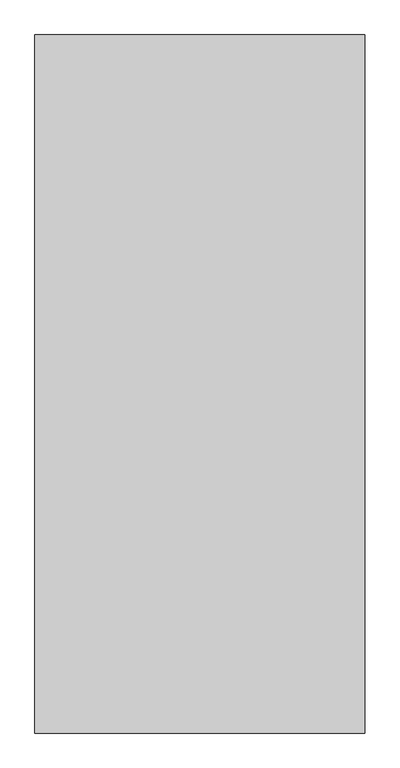
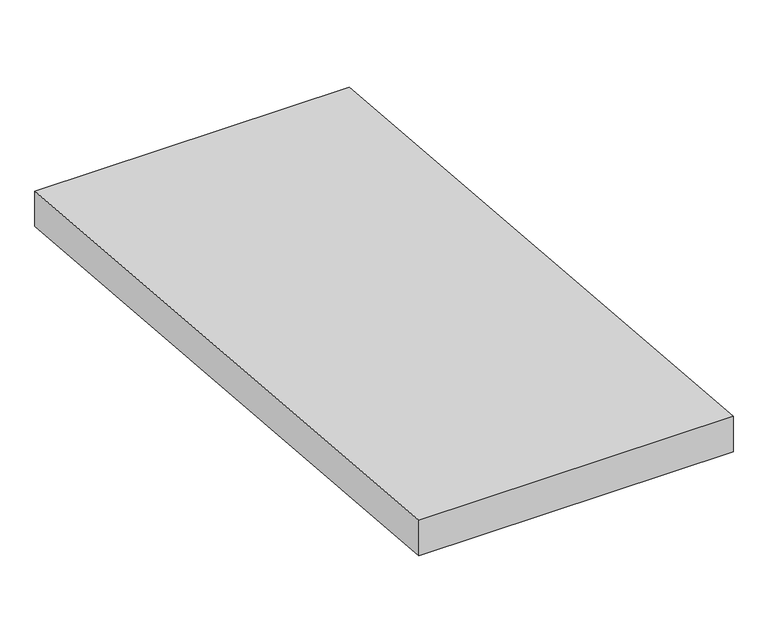
"""IFC4 building model written with IfcOpenShell, lengths in millimetres: ramp geometry."""

import ifcopenshell
import ifcopenshell.guid

model = None  # the IFC model being written
_history = None  # IfcOwnerHistory: only IFC2X3 demands one
_inside = {}  # id of a spatial element -> (the spatial element, [elements in it])
_under = {}  # id of a project, library or spatial element -> (it, [spatial elements below it])
_declared = {}  # id of a project -> (the project, [libraries it declares])
_typed = {}  # id of a type object -> (the type object, [elements of that type])
_made_of = {}  # id of a material, layer set ... -> (it, [elements and type objects made of it])


def new_model(schema):
    """Start an empty IFC model of exactly this schema.

    Asked for "IFC4X3", IfcOpenShell would pick the latest addendum, in which some entities
    have other attributes; the version numbers below select the first issue.
    IFC2X3 requires an IfcOwnerHistory on every rooted entity: one is made here for all.
    """
    global model, _history
    if schema == "IFC4X3":
        model = ifcopenshell.file(schema_version=(4, 3, 0, 0))
    else:
        model = ifcopenshell.file(schema=schema)
    _inside.clear()
    _under.clear()
    _declared.clear()
    _typed.clear()
    _made_of.clear()
    _history = None
    if model.schema == "IFC2X3":
        org = make("IfcOrganization", Name="unknown")
        user = make(
            "IfcPersonAndOrganization",
            ThePerson=make("IfcPerson", FamilyName="unknown"),
            TheOrganization=org,
        )
        app = make(
            "IfcApplication",
            ApplicationDeveloper=org,
            Version="unknown",
            ApplicationFullName="unknown",
            ApplicationIdentifier="unknown",
        )
        _history = make(
            "IfcOwnerHistory",
            OwningUser=user,
            OwningApplication=app,
            ChangeAction="ADDED",
            CreationDate=0,
        )
    return model


def make(cls, **values):
    """One entity of the class cls with the attributes given. An attribute that is None is left unset."""
    return model.create_entity(
        cls, **{name: value for name, value in values.items() if value is not None}
    )


def rooted(cls, **values):
    """An entity with a GlobalId (a new one), such as an element, a storey or a relation."""
    return make(cls, GlobalId=ifcopenshell.guid.new(), OwnerHistory=_history, **values)


def si_unit(unit_type, name, prefix=None):
    """IfcSIUnit, for example si_unit("LENGTHUNIT", "METRE", prefix="MILLI")."""
    return make("IfcSIUnit", UnitType=unit_type, Prefix=prefix, Name=name)


def assignment(units):
    """IfcUnitAssignment: the units of a project."""
    return None if units is None else make("IfcUnitAssignment", Units=units)


def point(xyz):
    """IfcCartesianPoint."""
    return None if xyz is None else make("IfcCartesianPoint", Coordinates=xyz)


def direction(xyz):
    """IfcDirection."""
    return None if xyz is None else make("IfcDirection", DirectionRatios=xyz)


def frame(location, z_axis=None, x_axis=None):
    """IfcAxis2Placement3D, a coordinate frame: its origin and axes. An axis left out is left unset."""
    return make(
        "IfcAxis2Placement3D",
        Location=point(location),
        Axis=direction(z_axis),
        RefDirection=direction(x_axis),
    )


def origin():
    """The frame at (0, 0, 0) with its axes left unset."""
    return frame((0.0, 0.0, 0.0))


def place(relative_to, where):
    """IfcLocalPlacement: puts the frame where relative to a parent placement (None: the world)."""
    return make(
        "IfcLocalPlacement", PlacementRelTo=relative_to, RelativePlacement=where
    )


def context(
    kind, dimensions, precision=None, world=None, true_north=None, identifier=None
):
    """IfcGeometricRepresentationContext, for example the 3D "Model" context."""
    return make(
        "IfcGeometricRepresentationContext",
        ContextIdentifier=identifier,
        ContextType=kind,
        CoordinateSpaceDimension=dimensions,
        Precision=precision,
        WorldCoordinateSystem=world,
        TrueNorth=true_north,
    )


def project(units=None, contexts=None):
    """IfcProject with its units and contexts."""
    return rooted(
        "IfcProject",
        Name="project",
        RepresentationContexts=contexts,
        UnitsInContext=assignment(units),
    )


def spatial(cls, under=None, at=None, **own):
    """A site, building, storey or space (cls), placed at a placement, below another one or the project."""
    s = rooted(cls, ObjectPlacement=at, **own)
    if under is not None:
        _under.setdefault(under.id(), (under, []))[1].append(s)
    return s


def polyline(points):
    """IfcPolyline through the points."""
    return make("IfcPolyline", Points=[point(p) for p in points])


def outline(outer, holes=None, kind="AREA"):
    """IfcArbitraryClosedProfileDef: a profile drawn as a closed curve; with holes, ...WithVoids."""
    if holes is None:
        return make("IfcArbitraryClosedProfileDef", ProfileType=kind, OuterCurve=outer)
    return make(
        "IfcArbitraryProfileDefWithVoids",
        ProfileType=kind,
        OuterCurve=outer,
        InnerCurves=holes,
    )


def extrude(swept, where, along, depth):
    """IfcExtrudedAreaSolid: the profile swept, set in the frame where, extruded along a direction by depth."""
    return make(
        "IfcExtrudedAreaSolid",
        SweptArea=swept,
        Position=where,
        ExtrudedDirection=direction(along),
        Depth=depth,
    )


def shape(context_of_items, identifier, shape_type, items):
    """IfcShapeRepresentation: the items that make up one representation, for example the "Body"."""
    return make(
        "IfcShapeRepresentation",
        ContextOfItems=context_of_items,
        RepresentationIdentifier=identifier,
        RepresentationType=shape_type,
        Items=items,
    )


def source(mapping_origin, context_of_items, identifier, shape_type, items):
    """IfcRepresentationMap: a shape defined once, which mapped items show again and again."""
    return make(
        "IfcRepresentationMap",
        MappingOrigin=mapping_origin,
        MappedRepresentation=shape(context_of_items, identifier, shape_type, items),
    )


def transform(
    local_origin,
    x_axis=None,
    y_axis=None,
    z_axis=None,
    scale=None,
    scale2=None,
    scale3=None,
    uniform=True,
):
    """IfcCartesianTransformationOperator3D, or its non-uniform kind. x_axis, y_axis, z_axis: its Axis1, 2, 3."""
    if uniform:
        return make(
            "IfcCartesianTransformationOperator3D",
            Axis1=direction(x_axis),
            Axis2=direction(y_axis),
            LocalOrigin=point(local_origin),
            Scale=scale,
            Axis3=direction(z_axis),
        )
    return make(
        "IfcCartesianTransformationOperator3DnonUniform",
        Axis1=direction(x_axis),
        Axis2=direction(y_axis),
        LocalOrigin=point(local_origin),
        Scale=scale,
        Axis3=direction(z_axis),
        Scale2=scale2,
        Scale3=scale3,
    )


def mapped(mapping_source, mapping_target):
    """IfcMappedItem: shows the shape of a source again, moved by a transform."""
    return make(
        "IfcMappedItem", MappingSource=mapping_source, MappingTarget=mapping_target
    )


def made_of(thing, what):
    """Note that an element or type object is made of a material, layer set ...; save() writes the relation."""
    if what is not None:
        _made_of.setdefault(what.id(), (what, []))[1].append(thing)
    return thing


def element(
    cls,
    number,
    at=None,
    inside=None,
    cuts=None,
    type_object=None,
    material=None,
    context=None,
    identifier="Body",
    shape_type=None,
    held_by="IfcProductDefinitionShape",
    body=None,
    shapes=None,
    **own,
):
    """One element of the class cls, such as IfcWall. Its Tag is "e" and its number.

    at: its placement. inside: the storey or other place that contains it. cuts: it is an
    opening in that element (IfcRelVoidsElement). A single representation is given by context,
    identifier, shape_type and body (its items); several are given by shapes. held_by: the class
    of the entity that holds the representations. save() writes the other relations.
    """
    e = rooted(cls, Tag="e%d" % number, ObjectPlacement=at, **own)
    if body is not None:
        shapes = [shape(context, identifier, shape_type, body)]
    if shapes is not None:
        e.Representation = make(held_by, Representations=shapes)
    if inside is not None:
        _inside.setdefault(inside.id(), (inside, []))[1].append(e)
    if cuts is not None:
        rooted(
            "IfcRelVoidsElement", RelatingBuildingElement=cuts, RelatedOpeningElement=e
        )
    if type_object is not None:
        _typed.setdefault(type_object.id(), (type_object, []))[1].append(e)
    return made_of(e, material)


def aggregate(whole, parts):
    """IfcRelAggregates: a whole, such as a stair, and the parts it consists of."""
    return rooted("IfcRelAggregates", RelatingObject=whole, RelatedObjects=parts)


def save(model, path):
    """Write the relations noted so far, then the file.

    IfcRelAggregates (storeys below a building ...), IfcRelContainedInSpatialStructure (elements
    in a storey), IfcRelDefinesByType, IfcRelAssociatesMaterial and IfcRelDeclares: one each for
    every whole, place, type object, material and project.
    """
    for whole, parts in _under.values():
        aggregate(whole, parts)
    for where, things in _inside.values():
        rooted(
            "IfcRelContainedInSpatialStructure",
            RelatedElements=things,
            RelatingStructure=where,
        )
    for kind, things in _typed.values():
        rooted("IfcRelDefinesByType", RelatedObjects=things, RelatingType=kind)
    for what, things in _made_of.values():
        rooted("IfcRelAssociatesMaterial", RelatedObjects=things, RelatingMaterial=what)
    for by, libraries in _declared.values():
        rooted("IfcRelDeclares", RelatingContext=by, RelatedDefinitions=libraries)
    model.write(path)


def ramp_d010aea3(model_context):
    return source(origin(), model_context, "Body", "SweptSolid", [
        extrude(outline(polyline([(19399.5208589, 149.9618634), (22999.5208589, -150.0381366), (22999.5208589, -350.7313796), (19399.5208589, -50.7313796), (19399.5208589, 149.9618634)])), frame((20675.0, 0.0, 0.0), z_axis=(1.0, 0.0, 0.0), x_axis=(0.0, 1.0, 0.0)), (0.0, 0.0, 1.0), 1700.0),
    ])


if __name__ == "__main__":
    model = new_model("IFC4")
    model_context = context("Model", 3, world=origin())
    ifc_project = project(units=[si_unit("LENGTHUNIT", "METRE", prefix="MILLI")], contexts=[model_context])
    site = spatial("IfcSite", under=ifc_project)
    building = spatial("IfcBuilding", under=site)
    placement = place(None, origin())
    ramp_shape = ramp_d010aea3(model_context)
    element("IfcRamp", 1, at=placement, inside=building, context=model_context, shape_type="MappedRepresentation", body=[
        mapped(ramp_shape, transform((0.0, 0.0, 0.0), x_axis=(1.0, 0.0, 0.0), y_axis=(0.0, 1.0, 0.0), z_axis=(0.0, 0.0, 1.0))),
    ])
    save(model, "model.ifc")

# Revit data of these elements
# Element 1 (IfcRamp)
#   Materials on its faces: "00_Concrete_Reinf. Conc."
# Materials
#   "00_Concrete_Reinf. Conc.": class "Concrete", colour RGB 176 176 176, transparency 0, Description = "Reinf. Conc.", Cost = 0, Image = Concrete.Cast-In-Place.Flat.Polished.Grey.jpg
